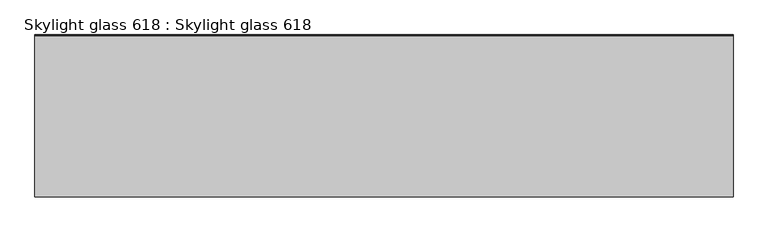
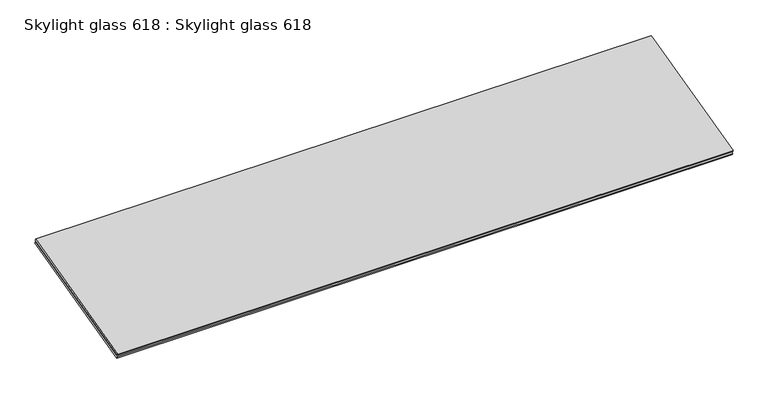
"""IFC4 building model written with IfcOpenShell, lengths in millimetres: proxy geometry, Skylight glass 618 : Skylight glass 618."""

from ifc_helpers import new_model, si_unit, frame, origin, place, context, project, spatial, polyline, outline, extrude, source, transform, mapped, element, save


def skylight_glass_618_skylight_glass_618_9c3f357c(model_context):
    return source(origin(), model_context, "Body", "SweptSolid", [
        extrude(outline(polyline([(9633.4400538, 43788.1259916), (9632.3198258, 43792.6038351), (10093.7955598, 43908.0518299), (10094.9379691, 43903.4853224), (9633.4400538, 43788.1259916)])), frame((3694.2883192, 0.0, 0.0), z_axis=(1.0, 0.0, 0.0), x_axis=(0.0, 1.0, 0.0)), (0.0, 0.0, 1.0), 2000.0),
        extrude(outline(polyline([(9630.4722335, 43799.942238), (9629.3741867, 43804.3314175), (10090.8609639, 43919.782175), (10091.9811919, 43915.3043315), (9630.4722335, 43799.942238)])), frame((3694.2883192, 0.0, 0.0), z_axis=(1.0, 0.0, 0.0), x_axis=(0.0, 1.0, 0.0)), (0.0, 0.0, 1.0), 2000.0),
    ])


if __name__ == "__main__":
    model = new_model("IFC4")
    model_context = context("Model", 3, world=origin())
    ifc_project = project(units=[si_unit("LENGTHUNIT", "METRE", prefix="MILLI")], contexts=[model_context])
    site = spatial("IfcSite", under=ifc_project)
    building = spatial("IfcBuilding", under=site)
    placement = place(None, origin())
    skylight_glass_618_skylight_glass_618_shape = skylight_glass_618_skylight_glass_618_9c3f357c(model_context)
    element("IfcBuildingElementProxy", 1, Name="Skylight glass 618 : Skylight glass 618", ObjectType="Skylight glass 618 : Skylight glass 618", at=placement, inside=building, context=model_context, shape_type="MappedRepresentation", body=[
        mapped(skylight_glass_618_skylight_glass_618_shape, transform((0.0, 0.0, 0.0), x_axis=(1.0, 0.0, 0.0), y_axis=(0.0, 1.0, 0.0), z_axis=(0.0, 0.0, 1.0))),
    ])
    save(model, "model.ifc")

# Revit data of these elements
# Type "Skylight glass 618 : Skylight glass 618"
#   NameOverride = "Skylight glass"
# Element 1 (IfcBuildingElementProxy, "Skylight glass 618 : Skylight glass 618")
#   Materials on its faces: "1\"  INSULATED GLAZING"
# Materials
#   "1\"  INSULATED GLAZING": class "Unassigned", colour RGB 146 199 212, transparency 0, Cost = 0
